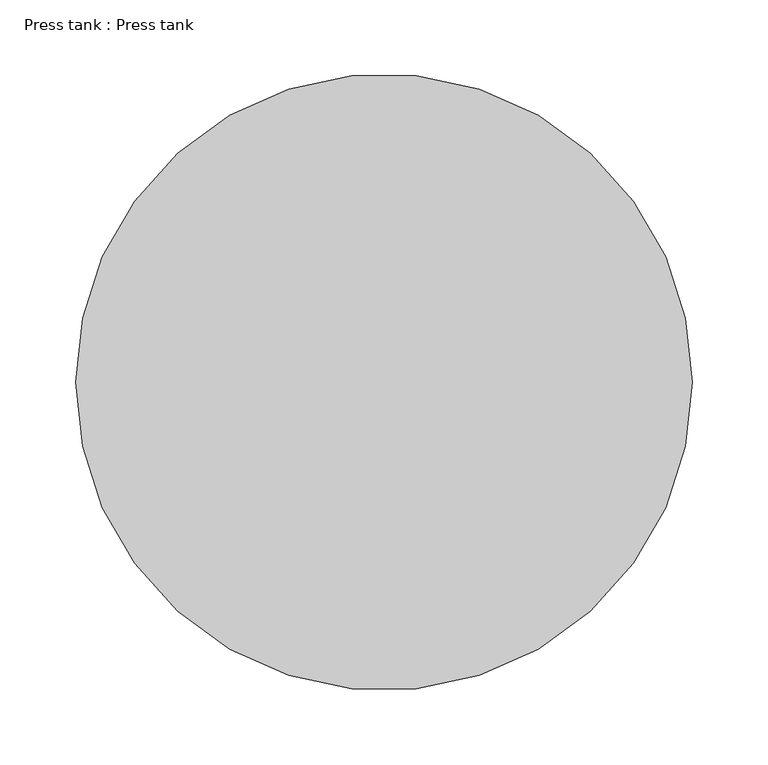
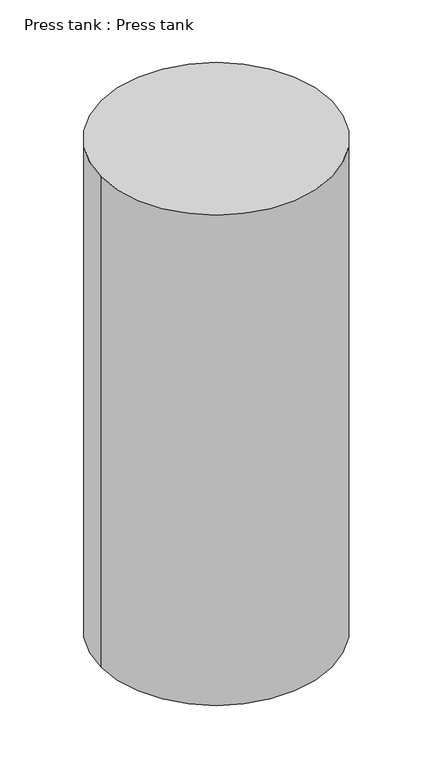
"""IFC4 building model written with IfcOpenShell, lengths in millimetres: proxy geometry, Press tank : Press tank."""

import ifcopenshell
import ifcopenshell.guid

model = None  # the IFC model being written
_history = None  # IfcOwnerHistory: only IFC2X3 demands one
_inside = {}  # id of a spatial element -> (the spatial element, [elements in it])
_under = {}  # id of a project, library or spatial element -> (it, [spatial elements below it])
_declared = {}  # id of a project -> (the project, [libraries it declares])
_typed = {}  # id of a type object -> (the type object, [elements of that type])
_made_of = {}  # id of a material, layer set ... -> (it, [elements and type objects made of it])


def new_model(schema):
    """Start an empty IFC model of exactly this schema.

    Asked for "IFC4X3", IfcOpenShell would pick the latest addendum, in which some entities
    have other attributes; the version numbers below select the first issue.
    IFC2X3 requires an IfcOwnerHistory on every rooted entity: one is made here for all.
    """
    global model, _history
    if schema == "IFC4X3":
        model = ifcopenshell.file(schema_version=(4, 3, 0, 0))
    else:
        model = ifcopenshell.file(schema=schema)
    _inside.clear()
    _under.clear()
    _declared.clear()
    _typed.clear()
    _made_of.clear()
    _history = None
    if model.schema == "IFC2X3":
        org = make("IfcOrganization", Name="unknown")
        user = make(
            "IfcPersonAndOrganization",
            ThePerson=make("IfcPerson", FamilyName="unknown"),
            TheOrganization=org,
        )
        app = make(
            "IfcApplication",
            ApplicationDeveloper=org,
            Version="unknown",
            ApplicationFullName="unknown",
            ApplicationIdentifier="unknown",
        )
        _history = make(
            "IfcOwnerHistory",
            OwningUser=user,
            OwningApplication=app,
            ChangeAction="ADDED",
            CreationDate=0,
        )
    return model


def make(cls, **values):
    """One entity of the class cls with the attributes given. An attribute that is None is left unset."""
    return model.create_entity(
        cls, **{name: value for name, value in values.items() if value is not None}
    )


def rooted(cls, **values):
    """An entity with a GlobalId (a new one), such as an element, a storey or a relation."""
    return make(cls, GlobalId=ifcopenshell.guid.new(), OwnerHistory=_history, **values)


def si_unit(unit_type, name, prefix=None):
    """IfcSIUnit, for example si_unit("LENGTHUNIT", "METRE", prefix="MILLI")."""
    return make("IfcSIUnit", UnitType=unit_type, Prefix=prefix, Name=name)


def assignment(units):
    """IfcUnitAssignment: the units of a project."""
    return None if units is None else make("IfcUnitAssignment", Units=units)


def point(xyz):
    """IfcCartesianPoint."""
    return None if xyz is None else make("IfcCartesianPoint", Coordinates=xyz)


def direction(xyz):
    """IfcDirection."""
    return None if xyz is None else make("IfcDirection", DirectionRatios=xyz)


def frame(location, z_axis=None, x_axis=None):
    """IfcAxis2Placement3D, a coordinate frame: its origin and axes. An axis left out is left unset."""
    return make(
        "IfcAxis2Placement3D",
        Location=point(location),
        Axis=direction(z_axis),
        RefDirection=direction(x_axis),
    )


def frame_2d(location, x_axis=None):
    """IfcAxis2Placement2D, a coordinate frame in the plane: its origin and x axis."""
    return make(
        "IfcAxis2Placement2D", Location=point(location), RefDirection=direction(x_axis)
    )


def origin():
    """The frame at (0, 0, 0) with its axes left unset."""
    return frame((0.0, 0.0, 0.0))


def place(relative_to, where):
    """IfcLocalPlacement: puts the frame where relative to a parent placement (None: the world)."""
    return make(
        "IfcLocalPlacement", PlacementRelTo=relative_to, RelativePlacement=where
    )


def context(
    kind, dimensions, precision=None, world=None, true_north=None, identifier=None
):
    """IfcGeometricRepresentationContext, for example the 3D "Model" context."""
    return make(
        "IfcGeometricRepresentationContext",
        ContextIdentifier=identifier,
        ContextType=kind,
        CoordinateSpaceDimension=dimensions,
        Precision=precision,
        WorldCoordinateSystem=world,
        TrueNorth=true_north,
    )


def project(units=None, contexts=None):
    """IfcProject with its units and contexts."""
    return rooted(
        "IfcProject",
        Name="project",
        RepresentationContexts=contexts,
        UnitsInContext=assignment(units),
    )


def spatial(cls, under=None, at=None, **own):
    """A site, building, storey or space (cls), placed at a placement, below another one or the project."""
    s = rooted(cls, ObjectPlacement=at, **own)
    if under is not None:
        _under.setdefault(under.id(), (under, []))[1].append(s)
    return s


def circle_curve(where, radius):
    """IfcCircle in the frame where."""
    return make("IfcCircle", Position=where, Radius=radius)


def trimmed(basis, trim1, trim2, sense, master):
    """IfcTrimmedCurve: the piece of a basis curve between two trims."""
    return make(
        "IfcTrimmedCurve",
        BasisCurve=basis,
        Trim1=trim1,
        Trim2=trim2,
        SenseAgreement=sense,
        MasterRepresentation=master,
    )


def segment(curve, same_sense, transition):
    """IfcCompositeCurveSegment."""
    return make(
        "IfcCompositeCurveSegment",
        Transition=transition,
        SameSense=same_sense,
        ParentCurve=curve,
    )


def composite_curve(segments, self_intersect=None):
    """IfcCompositeCurve: segments joined end to end."""
    return make("IfcCompositeCurve", Segments=segments, SelfIntersect=self_intersect)


def outline(outer, holes=None, kind="AREA"):
    """IfcArbitraryClosedProfileDef: a profile drawn as a closed curve; with holes, ...WithVoids."""
    if holes is None:
        return make("IfcArbitraryClosedProfileDef", ProfileType=kind, OuterCurve=outer)
    return make(
        "IfcArbitraryProfileDefWithVoids",
        ProfileType=kind,
        OuterCurve=outer,
        InnerCurves=holes,
    )


def extrude(swept, where, along, depth):
    """IfcExtrudedAreaSolid: the profile swept, set in the frame where, extruded along a direction by depth."""
    return make(
        "IfcExtrudedAreaSolid",
        SweptArea=swept,
        Position=where,
        ExtrudedDirection=direction(along),
        Depth=depth,
    )


def shape(context_of_items, identifier, shape_type, items):
    """IfcShapeRepresentation: the items that make up one representation, for example the "Body"."""
    return make(
        "IfcShapeRepresentation",
        ContextOfItems=context_of_items,
        RepresentationIdentifier=identifier,
        RepresentationType=shape_type,
        Items=items,
    )


def source(mapping_origin, context_of_items, identifier, shape_type, items):
    """IfcRepresentationMap: a shape defined once, which mapped items show again and again."""
    return make(
        "IfcRepresentationMap",
        MappingOrigin=mapping_origin,
        MappedRepresentation=shape(context_of_items, identifier, shape_type, items),
    )


def transform(
    local_origin,
    x_axis=None,
    y_axis=None,
    z_axis=None,
    scale=None,
    scale2=None,
    scale3=None,
    uniform=True,
):
    """IfcCartesianTransformationOperator3D, or its non-uniform kind. x_axis, y_axis, z_axis: its Axis1, 2, 3."""
    if uniform:
        return make(
            "IfcCartesianTransformationOperator3D",
            Axis1=direction(x_axis),
            Axis2=direction(y_axis),
            LocalOrigin=point(local_origin),
            Scale=scale,
            Axis3=direction(z_axis),
        )
    return make(
        "IfcCartesianTransformationOperator3DnonUniform",
        Axis1=direction(x_axis),
        Axis2=direction(y_axis),
        LocalOrigin=point(local_origin),
        Scale=scale,
        Axis3=direction(z_axis),
        Scale2=scale2,
        Scale3=scale3,
    )


def mapped(mapping_source, mapping_target):
    """IfcMappedItem: shows the shape of a source again, moved by a transform."""
    return make(
        "IfcMappedItem", MappingSource=mapping_source, MappingTarget=mapping_target
    )


def made_of(thing, what):
    """Note that an element or type object is made of a material, layer set ...; save() writes the relation."""
    if what is not None:
        _made_of.setdefault(what.id(), (what, []))[1].append(thing)
    return thing


def element(
    cls,
    number,
    at=None,
    inside=None,
    cuts=None,
    type_object=None,
    material=None,
    context=None,
    identifier="Body",
    shape_type=None,
    held_by="IfcProductDefinitionShape",
    body=None,
    shapes=None,
    **own,
):
    """One element of the class cls, such as IfcWall. Its Tag is "e" and its number.

    at: its placement. inside: the storey or other place that contains it. cuts: it is an
    opening in that element (IfcRelVoidsElement). A single representation is given by context,
    identifier, shape_type and body (its items); several are given by shapes. held_by: the class
    of the entity that holds the representations. save() writes the other relations.
    """
    e = rooted(cls, Tag="e%d" % number, ObjectPlacement=at, **own)
    if body is not None:
        shapes = [shape(context, identifier, shape_type, body)]
    if shapes is not None:
        e.Representation = make(held_by, Representations=shapes)
    if inside is not None:
        _inside.setdefault(inside.id(), (inside, []))[1].append(e)
    if cuts is not None:
        rooted(
            "IfcRelVoidsElement", RelatingBuildingElement=cuts, RelatedOpeningElement=e
        )
    if type_object is not None:
        _typed.setdefault(type_object.id(), (type_object, []))[1].append(e)
    return made_of(e, material)


def aggregate(whole, parts):
    """IfcRelAggregates: a whole, such as a stair, and the parts it consists of."""
    return rooted("IfcRelAggregates", RelatingObject=whole, RelatedObjects=parts)


def save(model, path):
    """Write the relations noted so far, then the file.

    IfcRelAggregates (storeys below a building ...), IfcRelContainedInSpatialStructure (elements
    in a storey), IfcRelDefinesByType, IfcRelAssociatesMaterial and IfcRelDeclares: one each for
    every whole, place, type object, material and project.
    """
    for whole, parts in _under.values():
        aggregate(whole, parts)
    for where, things in _inside.values():
        rooted(
            "IfcRelContainedInSpatialStructure",
            RelatedElements=things,
            RelatingStructure=where,
        )
    for kind, things in _typed.values():
        rooted("IfcRelDefinesByType", RelatedObjects=things, RelatingType=kind)
    for what, things in _made_of.values():
        rooted("IfcRelAssociatesMaterial", RelatedObjects=things, RelatingMaterial=what)
    for by, libraries in _declared.values():
        rooted("IfcRelDeclares", RelatingContext=by, RelatedDefinitions=libraries)
    model.write(path)


def press_tank_press_tank_b5f43448(model_context):
    return source(origin(), model_context, "Body", "SweptSolid", [
        extrude(outline(composite_curve([segment(trimmed(circle_curve(frame_2d((23819.6370052, 10524.1286841)), 203.2), [point((23616.4370052, 10524.1286841))], [point((24022.8370052, 10524.1286841))], False, "CARTESIAN"), True, "CONTINUOUS"), segment(trimmed(circle_curve(frame_2d((23819.6370052, 10524.1286841)), 203.2), [point((24022.8370052, 10524.1286841))], [point((23616.4370052, 10524.1286841))], False, "CARTESIAN"), True, "CONTINUOUS")], self_intersect=False)), frame((0.0, 0.0, 2832.1), z_axis=(0.0, 0.0, 1.0), x_axis=(1.0, 0.0, 0.0)), (0.0, 0.0, 1.0), 914.4),
    ])


if __name__ == "__main__":
    model = new_model("IFC4")
    model_context = context("Model", 3, world=origin())
    ifc_project = project(units=[si_unit("LENGTHUNIT", "METRE", prefix="MILLI")], contexts=[model_context])
    site = spatial("IfcSite", under=ifc_project)
    building = spatial("IfcBuilding", under=site)
    placement = place(None, origin())
    press_tank_press_tank_shape = press_tank_press_tank_b5f43448(model_context)
    element("IfcBuildingElementProxy", 1, Name="Press tank : Press tank", ObjectType="Press tank : Press tank", at=placement, inside=building, context=model_context, shape_type="MappedRepresentation", body=[
        mapped(press_tank_press_tank_shape, transform((0.0, 0.0, 0.0), x_axis=(1.0, 0.0, 0.0), y_axis=(0.0, 1.0, 0.0), z_axis=(0.0, 0.0, 1.0))),
    ])
    save(model, "model.ifc")
